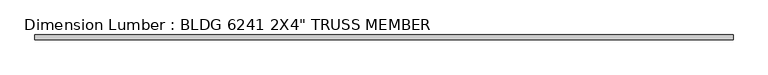
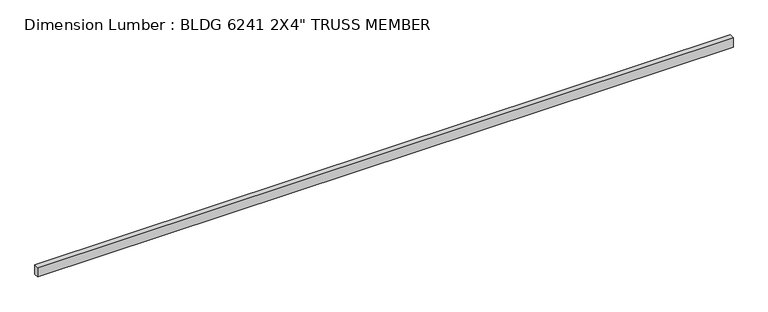
"""IFC4 building model written with IfcOpenShell, lengths in millimetres: beam geometry."""

import ifcopenshell
import ifcopenshell.guid

model = None  # the IFC model being written
_history = None  # IfcOwnerHistory: only IFC2X3 demands one
_inside = {}  # id of a spatial element -> (the spatial element, [elements in it])
_under = {}  # id of a project, library or spatial element -> (it, [spatial elements below it])
_declared = {}  # id of a project -> (the project, [libraries it declares])
_typed = {}  # id of a type object -> (the type object, [elements of that type])
_made_of = {}  # id of a material, layer set ... -> (it, [elements and type objects made of it])


def new_model(schema):
    """Start an empty IFC model of exactly this schema.

    Asked for "IFC4X3", IfcOpenShell would pick the latest addendum, in which some entities
    have other attributes; the version numbers below select the first issue.
    IFC2X3 requires an IfcOwnerHistory on every rooted entity: one is made here for all.
    """
    global model, _history
    if schema == "IFC4X3":
        model = ifcopenshell.file(schema_version=(4, 3, 0, 0))
    else:
        model = ifcopenshell.file(schema=schema)
    _inside.clear()
    _under.clear()
    _declared.clear()
    _typed.clear()
    _made_of.clear()
    _history = None
    if model.schema == "IFC2X3":
        org = make("IfcOrganization", Name="unknown")
        user = make(
            "IfcPersonAndOrganization",
            ThePerson=make("IfcPerson", FamilyName="unknown"),
            TheOrganization=org,
        )
        app = make(
            "IfcApplication",
            ApplicationDeveloper=org,
            Version="unknown",
            ApplicationFullName="unknown",
            ApplicationIdentifier="unknown",
        )
        _history = make(
            "IfcOwnerHistory",
            OwningUser=user,
            OwningApplication=app,
            ChangeAction="ADDED",
            CreationDate=0,
        )
    return model


def make(cls, **values):
    """One entity of the class cls with the attributes given. An attribute that is None is left unset."""
    return model.create_entity(
        cls, **{name: value for name, value in values.items() if value is not None}
    )


def rooted(cls, **values):
    """An entity with a GlobalId (a new one), such as an element, a storey or a relation."""
    return make(cls, GlobalId=ifcopenshell.guid.new(), OwnerHistory=_history, **values)


def si_unit(unit_type, name, prefix=None):
    """IfcSIUnit, for example si_unit("LENGTHUNIT", "METRE", prefix="MILLI")."""
    return make("IfcSIUnit", UnitType=unit_type, Prefix=prefix, Name=name)


def assignment(units):
    """IfcUnitAssignment: the units of a project."""
    return None if units is None else make("IfcUnitAssignment", Units=units)


def point(xyz):
    """IfcCartesianPoint."""
    return None if xyz is None else make("IfcCartesianPoint", Coordinates=xyz)


def direction(xyz):
    """IfcDirection."""
    return None if xyz is None else make("IfcDirection", DirectionRatios=xyz)


def frame(location, z_axis=None, x_axis=None):
    """IfcAxis2Placement3D, a coordinate frame: its origin and axes. An axis left out is left unset."""
    return make(
        "IfcAxis2Placement3D",
        Location=point(location),
        Axis=direction(z_axis),
        RefDirection=direction(x_axis),
    )


def origin():
    """The frame at (0, 0, 0) with its axes left unset."""
    return frame((0.0, 0.0, 0.0))


def place(relative_to, where):
    """IfcLocalPlacement: puts the frame where relative to a parent placement (None: the world)."""
    return make(
        "IfcLocalPlacement", PlacementRelTo=relative_to, RelativePlacement=where
    )


def context(
    kind, dimensions, precision=None, world=None, true_north=None, identifier=None
):
    """IfcGeometricRepresentationContext, for example the 3D "Model" context."""
    return make(
        "IfcGeometricRepresentationContext",
        ContextIdentifier=identifier,
        ContextType=kind,
        CoordinateSpaceDimension=dimensions,
        Precision=precision,
        WorldCoordinateSystem=world,
        TrueNorth=true_north,
    )


def project(units=None, contexts=None):
    """IfcProject with its units and contexts."""
    return rooted(
        "IfcProject",
        Name="project",
        RepresentationContexts=contexts,
        UnitsInContext=assignment(units),
    )


def spatial(cls, under=None, at=None, **own):
    """A site, building, storey or space (cls), placed at a placement, below another one or the project."""
    s = rooted(cls, ObjectPlacement=at, **own)
    if under is not None:
        _under.setdefault(under.id(), (under, []))[1].append(s)
    return s


def polyline(points):
    """IfcPolyline through the points."""
    return make("IfcPolyline", Points=[point(p) for p in points])


def outline(outer, holes=None, kind="AREA"):
    """IfcArbitraryClosedProfileDef: a profile drawn as a closed curve; with holes, ...WithVoids."""
    if holes is None:
        return make("IfcArbitraryClosedProfileDef", ProfileType=kind, OuterCurve=outer)
    return make(
        "IfcArbitraryProfileDefWithVoids",
        ProfileType=kind,
        OuterCurve=outer,
        InnerCurves=holes,
    )


def extrude(swept, where, along, depth):
    """IfcExtrudedAreaSolid: the profile swept, set in the frame where, extruded along a direction by depth."""
    return make(
        "IfcExtrudedAreaSolid",
        SweptArea=swept,
        Position=where,
        ExtrudedDirection=direction(along),
        Depth=depth,
    )


def shape(context_of_items, identifier, shape_type, items):
    """IfcShapeRepresentation: the items that make up one representation, for example the "Body"."""
    return make(
        "IfcShapeRepresentation",
        ContextOfItems=context_of_items,
        RepresentationIdentifier=identifier,
        RepresentationType=shape_type,
        Items=items,
    )


def source(mapping_origin, context_of_items, identifier, shape_type, items):
    """IfcRepresentationMap: a shape defined once, which mapped items show again and again."""
    return make(
        "IfcRepresentationMap",
        MappingOrigin=mapping_origin,
        MappedRepresentation=shape(context_of_items, identifier, shape_type, items),
    )


def transform(
    local_origin,
    x_axis=None,
    y_axis=None,
    z_axis=None,
    scale=None,
    scale2=None,
    scale3=None,
    uniform=True,
):
    """IfcCartesianTransformationOperator3D, or its non-uniform kind. x_axis, y_axis, z_axis: its Axis1, 2, 3."""
    if uniform:
        return make(
            "IfcCartesianTransformationOperator3D",
            Axis1=direction(x_axis),
            Axis2=direction(y_axis),
            LocalOrigin=point(local_origin),
            Scale=scale,
            Axis3=direction(z_axis),
        )
    return make(
        "IfcCartesianTransformationOperator3DnonUniform",
        Axis1=direction(x_axis),
        Axis2=direction(y_axis),
        LocalOrigin=point(local_origin),
        Scale=scale,
        Axis3=direction(z_axis),
        Scale2=scale2,
        Scale3=scale3,
    )


def mapped(mapping_source, mapping_target):
    """IfcMappedItem: shows the shape of a source again, moved by a transform."""
    return make(
        "IfcMappedItem", MappingSource=mapping_source, MappingTarget=mapping_target
    )


def made_of(thing, what):
    """Note that an element or type object is made of a material, layer set ...; save() writes the relation."""
    if what is not None:
        _made_of.setdefault(what.id(), (what, []))[1].append(thing)
    return thing


def element(
    cls,
    number,
    at=None,
    inside=None,
    cuts=None,
    type_object=None,
    material=None,
    context=None,
    identifier="Body",
    shape_type=None,
    held_by="IfcProductDefinitionShape",
    body=None,
    shapes=None,
    **own,
):
    """One element of the class cls, such as IfcWall. Its Tag is "e" and its number.

    at: its placement. inside: the storey or other place that contains it. cuts: it is an
    opening in that element (IfcRelVoidsElement). A single representation is given by context,
    identifier, shape_type and body (its items); several are given by shapes. held_by: the class
    of the entity that holds the representations. save() writes the other relations.
    """
    e = rooted(cls, Tag="e%d" % number, ObjectPlacement=at, **own)
    if body is not None:
        shapes = [shape(context, identifier, shape_type, body)]
    if shapes is not None:
        e.Representation = make(held_by, Representations=shapes)
    if inside is not None:
        _inside.setdefault(inside.id(), (inside, []))[1].append(e)
    if cuts is not None:
        rooted(
            "IfcRelVoidsElement", RelatingBuildingElement=cuts, RelatedOpeningElement=e
        )
    if type_object is not None:
        _typed.setdefault(type_object.id(), (type_object, []))[1].append(e)
    return made_of(e, material)


def aggregate(whole, parts):
    """IfcRelAggregates: a whole, such as a stair, and the parts it consists of."""
    return rooted("IfcRelAggregates", RelatingObject=whole, RelatedObjects=parts)


def save(model, path):
    """Write the relations noted so far, then the file.

    IfcRelAggregates (storeys below a building ...), IfcRelContainedInSpatialStructure (elements
    in a storey), IfcRelDefinesByType, IfcRelAssociatesMaterial and IfcRelDeclares: one each for
    every whole, place, type object, material and project.
    """
    for whole, parts in _under.values():
        aggregate(whole, parts)
    for where, things in _inside.values():
        rooted(
            "IfcRelContainedInSpatialStructure",
            RelatedElements=things,
            RelatingStructure=where,
        )
    for kind, things in _typed.values():
        rooted("IfcRelDefinesByType", RelatedObjects=things, RelatingType=kind)
    for what, things in _made_of.values():
        rooted("IfcRelAssociatesMaterial", RelatedObjects=things, RelatingMaterial=what)
    for by, libraries in _declared.values():
        rooted("IfcRelDeclares", RelatingContext=by, RelatedDefinitions=libraries)
    model.write(path)


def beam_38f3c654(model_context):
    return source(origin(), model_context, "Body", "SweptSolid", [
        extrude(outline(polyline([(3581.4, 25.4), (3581.4, -25.4), (-3556.0, -25.4), (-3556.0, 25.4), (3581.4, 25.4)])), frame((0.0, 0.0, -50.8), z_axis=(0.0, 0.0, 1.0), x_axis=(1.0, 0.0, 0.0)), (0.0, 0.0, 1.0), 101.6),
    ])


if __name__ == "__main__":
    model = new_model("IFC4")
    model_context = context("Model", 3, world=origin())
    ifc_project = project(units=[si_unit("LENGTHUNIT", "METRE", prefix="MILLI")], contexts=[model_context])
    site = spatial("IfcSite", under=ifc_project)
    building = spatial("IfcBuilding", under=site)
    placement = place(None, origin())
    beam_shape = beam_38f3c654(model_context)
    element("IfcBeam", 1, ObjectType="Dimension Lumber : BLDG 6241 2X4\" TRUSS MEMBER", at=placement, inside=building, context=model_context, shape_type="MappedRepresentation", body=[
        mapped(beam_shape, transform((0.0, 0.0, 0.0), x_axis=(1.0, 0.0, 0.0), y_axis=(0.0, 1.0, 0.0), z_axis=(0.0, 0.0, 1.0))),
    ])
    save(model, "model.ifc")

# Revit data of these elements
# Type "Dimension Lumber : BLDG 6241 2X4\" TRUSS MEMBER"
#   Assembly Code = "B10"
#   A = 0.273472 SF
#   Length [instance default] = 5' - 0"
#   b = 0' - 2"
#   d = 0' - 4"
#   Structural Material [instance default] = Softwood, Lumber
# Element 1 (IfcBeam, "Dimension Lumber : BLDG 6241 2X4\" TRUSS MEMBER")
#   Materials on its faces: "Softwood, Lumber"
# Materials
#   "Softwood, Lumber": class "Wood", colour RGB 223 192 134, transparency 0, Description = "Pinus Echinata", Cost = 0
